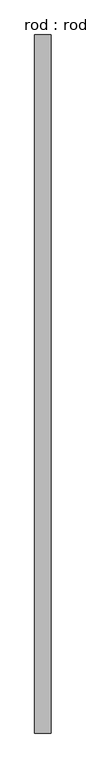
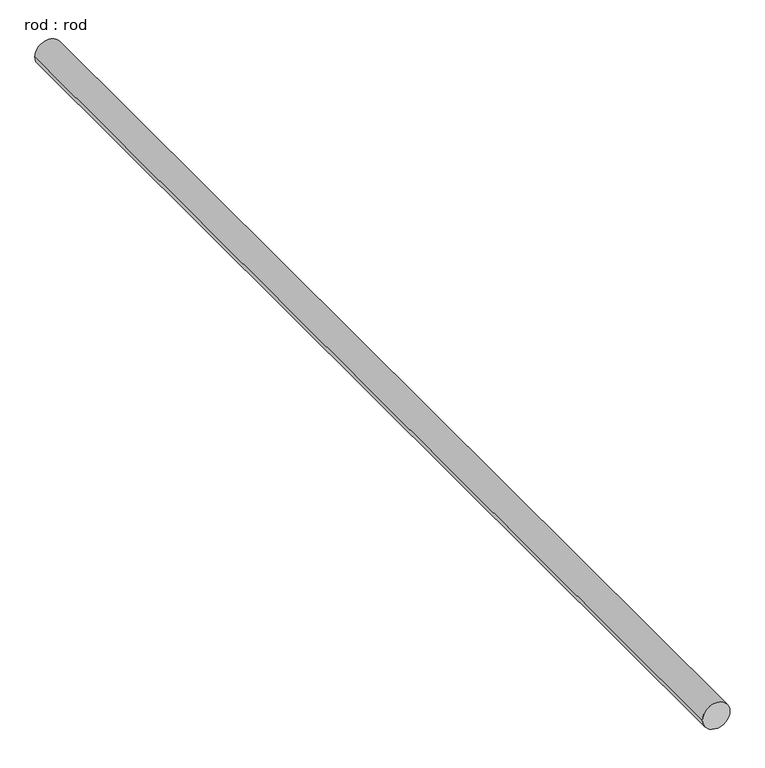
"""IFC4 building model written with IfcOpenShell, lengths in millimetres: proxy geometry, rod : rod."""

from ifc_helpers import new_model, si_unit, point, frame, frame_2d, origin, place, context, project, spatial, circle_curve, trimmed, segment, composite_curve, outline, extrude, source, transform, mapped, element, save


def rod_rod_c1da654d(model_context):
    return source(origin(), model_context, "Body", "SweptSolid", [
        extrude(outline(composite_curve([segment(trimmed(circle_curve(frame_2d((0.0108462, 0.0)), 200.0), [point((0.0108462, 200.0))], [point((0.0108462, -200.0))], False, "CARTESIAN"), True, "CONTINUOUS"), segment(trimmed(circle_curve(frame_2d((0.0108462, 0.0)), 200.0), [point((0.0108462, -200.0))], [point((0.0108462, 200.0))], False, "CARTESIAN"), True, "CONTINUOUS")], self_intersect=False)), frame((0.0, -4349.516164, 0.0), z_axis=(0.0, 1.0, 0.0), x_axis=(0.0, 0.0, 1.0)), (0.0, 0.0, 1.0), 16884.4895586),
    ])


if __name__ == "__main__":
    model = new_model("IFC4")
    model_context = context("Model", 3, world=origin())
    ifc_project = project(units=[si_unit("LENGTHUNIT", "METRE", prefix="MILLI")], contexts=[model_context])
    site = spatial("IfcSite", under=ifc_project)
    building = spatial("IfcBuilding", under=site)
    placement = place(None, origin())
    rod_rod_shape = rod_rod_c1da654d(model_context)
    element("IfcBuildingElementProxy", 1, Name="rod : rod", ObjectType="rod : rod", at=placement, inside=building, context=model_context, shape_type="MappedRepresentation", body=[
        mapped(rod_rod_shape, transform((0.0, 0.0, 0.0), x_axis=(1.0, 0.0, 0.0), y_axis=(0.0, 1.0, 0.0), z_axis=(0.0, 0.0, 1.0))),
    ])
    save(model, "model.ifc")

# Revit data of these elements
# Type "rod : rod"
#   Default Elevation = 0
